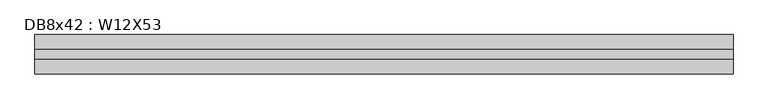
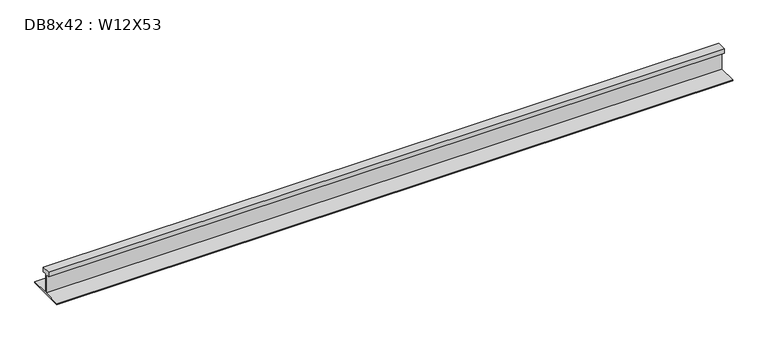
"""IFC4 building model written with IfcOpenShell, lengths in millimetres: beam geometry, DB8x42 : W12X53."""

from ifc_helpers import new_model, si_unit, frame, origin, place, context, project, spatial, polyline, outline, extrude, source, transform, mapped, element, save


def db8x42_w12x53_a2d98106(model_context):
    return source(origin(), model_context, "Body", "SweptSolid", [
        extrude(outline(polyline([(38.1, 144.3355), (38.1, 106.2355), (4.7625, 106.2355), (4.7625, -49.53), (152.4, -49.53), (152.4, -59.182), (-152.4, -59.182), (-152.4, -49.53), (-4.7625, -49.53), (-4.7625, 106.2355), (-38.1, 106.2355), (-38.1, 144.3355), (38.1, 144.3355)])), frame((-2708.529, 0.0, 0.0), z_axis=(1.0, 0.0, 0.0), x_axis=(0.0, 1.0, 0.0)), (0.0, 0.0, 1.0), 5417.058),
    ])


if __name__ == "__main__":
    model = new_model("IFC4")
    model_context = context("Model", 3, world=origin())
    ifc_project = project(units=[si_unit("LENGTHUNIT", "METRE", prefix="MILLI")], contexts=[model_context])
    site = spatial("IfcSite", under=ifc_project)
    building = spatial("IfcBuilding", under=site)
    placement = place(None, origin())
    db8x42_w12x53_shape = db8x42_w12x53_a2d98106(model_context)
    element("IfcBeam", 1, ObjectType="DB8x42 : W12X53", at=placement, inside=building, context=model_context, shape_type="MappedRepresentation", body=[
        mapped(db8x42_w12x53_shape, transform((0.0, 0.0, 0.0), x_axis=(1.0, 0.0, 0.0), y_axis=(0.0, 1.0, 0.0), z_axis=(0.0, 0.0, 1.0))),
    ])
    save(model, "model.ifc")

# Revit data of these elements
# Type "DB8x42 : W12X53"
#   Assembly Code = "B10"
#   W = 53
#   Length [instance default] = 5' - 0"
#   bf = 0' - 10"
#   d = 1' - 0.1"
#   k = 0' - 1 3/8"
#   k2 = 0' - 0.8"
#   tf = 0' - 0.575"
#   tw = 0' - 0.345"
#   A = 0.108333 SF
#   Structural Material [instance default] = Steel ASTM A992
# Element 1 (IfcBeam, "DB8x42 : W12X53")
#   Materials on its faces: "Steel ASTM A992"
# Materials
#   "Steel ASTM A992": class "Metal", colour RGB 199 199 199, transparency 0, Description = "Structural steel 50ksi", Cost = 0
